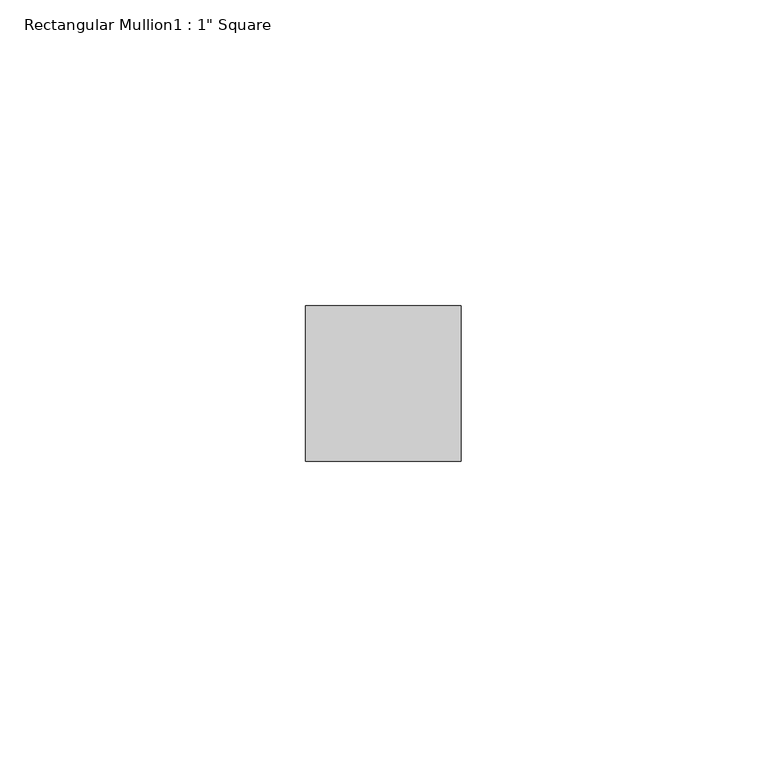
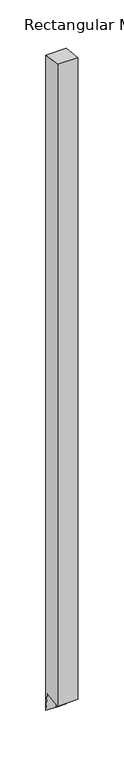
"""IFC4 building model written with IfcOpenShell, lengths in millimetres: member geometry."""

import ifcopenshell
import ifcopenshell.guid

model = None  # the IFC model being written
_history = None  # IfcOwnerHistory: only IFC2X3 demands one
_inside = {}  # id of a spatial element -> (the spatial element, [elements in it])
_under = {}  # id of a project, library or spatial element -> (it, [spatial elements below it])
_declared = {}  # id of a project -> (the project, [libraries it declares])
_typed = {}  # id of a type object -> (the type object, [elements of that type])
_made_of = {}  # id of a material, layer set ... -> (it, [elements and type objects made of it])


def new_model(schema):
    """Start an empty IFC model of exactly this schema.

    Asked for "IFC4X3", IfcOpenShell would pick the latest addendum, in which some entities
    have other attributes; the version numbers below select the first issue.
    IFC2X3 requires an IfcOwnerHistory on every rooted entity: one is made here for all.
    """
    global model, _history
    if schema == "IFC4X3":
        model = ifcopenshell.file(schema_version=(4, 3, 0, 0))
    else:
        model = ifcopenshell.file(schema=schema)
    _inside.clear()
    _under.clear()
    _declared.clear()
    _typed.clear()
    _made_of.clear()
    _history = None
    if model.schema == "IFC2X3":
        org = make("IfcOrganization", Name="unknown")
        user = make(
            "IfcPersonAndOrganization",
            ThePerson=make("IfcPerson", FamilyName="unknown"),
            TheOrganization=org,
        )
        app = make(
            "IfcApplication",
            ApplicationDeveloper=org,
            Version="unknown",
            ApplicationFullName="unknown",
            ApplicationIdentifier="unknown",
        )
        _history = make(
            "IfcOwnerHistory",
            OwningUser=user,
            OwningApplication=app,
            ChangeAction="ADDED",
            CreationDate=0,
        )
    return model


def make(cls, **values):
    """One entity of the class cls with the attributes given. An attribute that is None is left unset."""
    return model.create_entity(
        cls, **{name: value for name, value in values.items() if value is not None}
    )


def rooted(cls, **values):
    """An entity with a GlobalId (a new one), such as an element, a storey or a relation."""
    return make(cls, GlobalId=ifcopenshell.guid.new(), OwnerHistory=_history, **values)


def si_unit(unit_type, name, prefix=None):
    """IfcSIUnit, for example si_unit("LENGTHUNIT", "METRE", prefix="MILLI")."""
    return make("IfcSIUnit", UnitType=unit_type, Prefix=prefix, Name=name)


def assignment(units):
    """IfcUnitAssignment: the units of a project."""
    return None if units is None else make("IfcUnitAssignment", Units=units)


def point(xyz):
    """IfcCartesianPoint."""
    return None if xyz is None else make("IfcCartesianPoint", Coordinates=xyz)


def direction(xyz):
    """IfcDirection."""
    return None if xyz is None else make("IfcDirection", DirectionRatios=xyz)


def frame(location, z_axis=None, x_axis=None):
    """IfcAxis2Placement3D, a coordinate frame: its origin and axes. An axis left out is left unset."""
    return make(
        "IfcAxis2Placement3D",
        Location=point(location),
        Axis=direction(z_axis),
        RefDirection=direction(x_axis),
    )


def origin():
    """The frame at (0, 0, 0) with its axes left unset."""
    return frame((0.0, 0.0, 0.0))


def place(relative_to, where):
    """IfcLocalPlacement: puts the frame where relative to a parent placement (None: the world)."""
    return make(
        "IfcLocalPlacement", PlacementRelTo=relative_to, RelativePlacement=where
    )


def context(
    kind, dimensions, precision=None, world=None, true_north=None, identifier=None
):
    """IfcGeometricRepresentationContext, for example the 3D "Model" context."""
    return make(
        "IfcGeometricRepresentationContext",
        ContextIdentifier=identifier,
        ContextType=kind,
        CoordinateSpaceDimension=dimensions,
        Precision=precision,
        WorldCoordinateSystem=world,
        TrueNorth=true_north,
    )


def project(units=None, contexts=None):
    """IfcProject with its units and contexts."""
    return rooted(
        "IfcProject",
        Name="project",
        RepresentationContexts=contexts,
        UnitsInContext=assignment(units),
    )


def spatial(cls, under=None, at=None, **own):
    """A site, building, storey or space (cls), placed at a placement, below another one or the project."""
    s = rooted(cls, ObjectPlacement=at, **own)
    if under is not None:
        _under.setdefault(under.id(), (under, []))[1].append(s)
    return s


def faces_of(points, faces, orient=None, outer=None):
    """IfcFace entities. A face is a list of loops; a loop is a list of indices into points, from 0.

    orient and outer hold one flag for each loop. By default every Orientation is true, the
    first loop of a face is its IfcFaceOuterBound and the others are IfcFaceBound.
    """
    made = []
    for i, loops in enumerate(faces):
        bounds = []
        for j, loop in enumerate(loops):
            is_outer = j == 0 if outer is None else outer[i][j]
            bounds.append(
                make(
                    "IfcFaceOuterBound" if is_outer else "IfcFaceBound",
                    Bound=make("IfcPolyLoop", Polygon=[points[k] for k in loop]),
                    Orientation=True if orient is None else orient[i][j],
                )
            )
        made.append(make("IfcFace", Bounds=bounds))
    return made


def faceted_brep(points, faces, orient=None, outer=None, voids=None):
    """IfcFacetedBrep: a solid bounded by flat faces; with voids (closed shells), ...WithVoids."""
    shared = [point(p) for p in points]
    hull = make("IfcClosedShell", CfsFaces=faces_of(shared, faces, orient, outer))
    if voids is None:
        return make("IfcFacetedBrep", Outer=hull)
    return make(
        "IfcFacetedBrepWithVoids",
        Outer=hull,
        Voids=[
            make(cls, CfsFaces=faces_of(shared, fs, o, b)) for cls, fs, o, b in voids
        ],
    )


def shape(context_of_items, identifier, shape_type, items):
    """IfcShapeRepresentation: the items that make up one representation, for example the "Body"."""
    return make(
        "IfcShapeRepresentation",
        ContextOfItems=context_of_items,
        RepresentationIdentifier=identifier,
        RepresentationType=shape_type,
        Items=items,
    )


def source(mapping_origin, context_of_items, identifier, shape_type, items):
    """IfcRepresentationMap: a shape defined once, which mapped items show again and again."""
    return make(
        "IfcRepresentationMap",
        MappingOrigin=mapping_origin,
        MappedRepresentation=shape(context_of_items, identifier, shape_type, items),
    )


def transform(
    local_origin,
    x_axis=None,
    y_axis=None,
    z_axis=None,
    scale=None,
    scale2=None,
    scale3=None,
    uniform=True,
):
    """IfcCartesianTransformationOperator3D, or its non-uniform kind. x_axis, y_axis, z_axis: its Axis1, 2, 3."""
    if uniform:
        return make(
            "IfcCartesianTransformationOperator3D",
            Axis1=direction(x_axis),
            Axis2=direction(y_axis),
            LocalOrigin=point(local_origin),
            Scale=scale,
            Axis3=direction(z_axis),
        )
    return make(
        "IfcCartesianTransformationOperator3DnonUniform",
        Axis1=direction(x_axis),
        Axis2=direction(y_axis),
        LocalOrigin=point(local_origin),
        Scale=scale,
        Axis3=direction(z_axis),
        Scale2=scale2,
        Scale3=scale3,
    )


def mapped(mapping_source, mapping_target):
    """IfcMappedItem: shows the shape of a source again, moved by a transform."""
    return make(
        "IfcMappedItem", MappingSource=mapping_source, MappingTarget=mapping_target
    )


def made_of(thing, what):
    """Note that an element or type object is made of a material, layer set ...; save() writes the relation."""
    if what is not None:
        _made_of.setdefault(what.id(), (what, []))[1].append(thing)
    return thing


def element(
    cls,
    number,
    at=None,
    inside=None,
    cuts=None,
    type_object=None,
    material=None,
    context=None,
    identifier="Body",
    shape_type=None,
    held_by="IfcProductDefinitionShape",
    body=None,
    shapes=None,
    **own,
):
    """One element of the class cls, such as IfcWall. Its Tag is "e" and its number.

    at: its placement. inside: the storey or other place that contains it. cuts: it is an
    opening in that element (IfcRelVoidsElement). A single representation is given by context,
    identifier, shape_type and body (its items); several are given by shapes. held_by: the class
    of the entity that holds the representations. save() writes the other relations.
    """
    e = rooted(cls, Tag="e%d" % number, ObjectPlacement=at, **own)
    if body is not None:
        shapes = [shape(context, identifier, shape_type, body)]
    if shapes is not None:
        e.Representation = make(held_by, Representations=shapes)
    if inside is not None:
        _inside.setdefault(inside.id(), (inside, []))[1].append(e)
    if cuts is not None:
        rooted(
            "IfcRelVoidsElement", RelatingBuildingElement=cuts, RelatedOpeningElement=e
        )
    if type_object is not None:
        _typed.setdefault(type_object.id(), (type_object, []))[1].append(e)
    return made_of(e, material)


def aggregate(whole, parts):
    """IfcRelAggregates: a whole, such as a stair, and the parts it consists of."""
    return rooted("IfcRelAggregates", RelatingObject=whole, RelatedObjects=parts)


def save(model, path):
    """Write the relations noted so far, then the file.

    IfcRelAggregates (storeys below a building ...), IfcRelContainedInSpatialStructure (elements
    in a storey), IfcRelDefinesByType, IfcRelAssociatesMaterial and IfcRelDeclares: one each for
    every whole, place, type object, material and project.
    """
    for whole, parts in _under.values():
        aggregate(whole, parts)
    for where, things in _inside.values():
        rooted(
            "IfcRelContainedInSpatialStructure",
            RelatedElements=things,
            RelatingStructure=where,
        )
    for kind, things in _typed.values():
        rooted("IfcRelDefinesByType", RelatedObjects=things, RelatingType=kind)
    for what, things in _made_of.values():
        rooted("IfcRelAssociatesMaterial", RelatedObjects=things, RelatingMaterial=what)
    for by, libraries in _declared.values():
        rooted("IfcRelDeclares", RelatingContext=by, RelatedDefinitions=libraries)
    model.write(path)


def member_b6f680d5(model_context):
    return source(origin(), model_context, "Body", "Brep", [
        faceted_brep([(-12.7, -19.05, 2.4841126), (12.7, -19.05, 2.4841126), (12.7, -19.05, -867.4148084), (0.0, -19.05, -867.4148084), (-12.7, -19.05, -867.4148084), (-12.7, -44.45, 5.7962627), (-12.7, -22.1744172, -843.4544818), (-12.7, -44.45, -846.3592091), (12.7, -44.45, 5.7962627), (0.0, -44.45, -846.3592091), (12.7, -44.45, -846.3592091), (12.7, -22.1744172, -843.4544818), (0.0, -22.1744172, -843.4544818)], [[[0, 1, 2, 3, 4]], [[5, 0, 4, 6, 7]], [[8, 5, 7, 9, 10]], [[1, 8, 10, 11, 2]], [[1, 0, 5, 8]], [[2, 11, 12, 3]], [[11, 10, 9, 12]], [[9, 7, 6, 12]], [[6, 4, 3, 12]]]),
    ])


if __name__ == "__main__":
    model = new_model("IFC4")
    model_context = context("Model", 3, world=origin())
    ifc_project = project(units=[si_unit("LENGTHUNIT", "METRE", prefix="MILLI")], contexts=[model_context])
    site = spatial("IfcSite", under=ifc_project)
    building = spatial("IfcBuilding", under=site)
    placement = place(None, origin())
    member_shape = member_b6f680d5(model_context)
    element("IfcMember", 1, ObjectType="Rectangular Mullion1 : 1\" Square", at=placement, inside=building, context=model_context, shape_type="MappedRepresentation", body=[
        mapped(member_shape, transform((0.0, 0.0, 0.0), x_axis=(1.0, 0.0, 0.0), y_axis=(0.0, 1.0, 0.0), z_axis=(0.0, 0.0, 1.0))),
    ])
    save(model, "model.ifc")

# Revit data of these elements
# Type "Rectangular Mullion1 : 1\" Square"
#   built-in parameter 1007351 = 0.104167 (stored number, unit not read)
#   built-in parameter 1007304 = 0.0833333 (stored number, unit not read)
#   built-in parameter 1007301 = 0.0416667 (stored number, unit not read)
#   built-in parameter 1007300 = 0.0416667 (stored number, unit not read)
